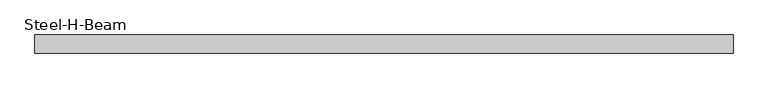
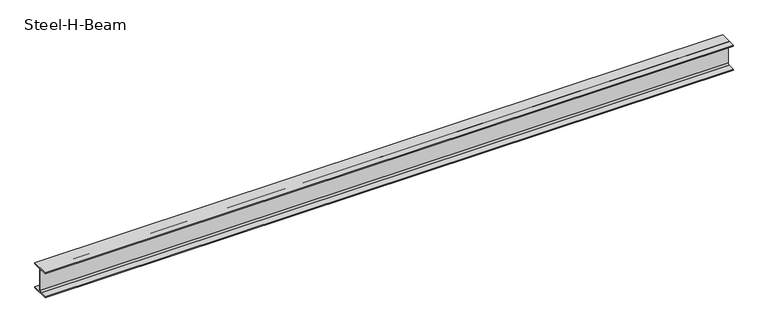
"""IFC4 building model written with IfcOpenShell, lengths in millimetres: beam geometry, Steel-H-Beam : BM121_H-294×200x8x12."""

from ifc_helpers import new_model, si_unit, point, frame, frame_2d, origin, place, context, project, spatial, polyline, circle_curve, trimmed, segment, composite_curve, outline, extrude, source, transform, mapped, element, save


def steel_h_beam_092dc31f(model_context):
    return source(origin(), model_context, "Body", "SweptSolid", [
        extrude(outline(composite_curve([segment(polyline([(100.0, -135.0), (100.0, -147.0), (-100.0, -147.0), (-100.0, -135.0), (-22.0, -135.0)]), True, "CONTINUOUS"), segment(trimmed(circle_curve(frame_2d((-22.0, -117.0)), 18.0), [point((-22.0, -135.0))], [point((-4.0, -117.0))], True, "CARTESIAN"), True, "CONTINUOUS"), segment(polyline([(-4.0, -117.0), (-4.0, 117.0)]), True, "CONTINUOUS"), segment(trimmed(circle_curve(frame_2d((-22.0, 117.0)), 18.0), [point((-4.0, 117.0))], [point((-22.0, 135.0))], True, "CARTESIAN"), True, "CONTINUOUS"), segment(polyline([(-22.0, 135.0), (-100.0, 135.0), (-100.0, 147.0), (100.0, 147.0), (100.0, 135.0), (22.0, 135.0)]), True, "CONTINUOUS"), segment(trimmed(circle_curve(frame_2d((22.0, 117.0)), 18.0), [point((22.0, 135.0))], [point((4.0, 117.0))], True, "CARTESIAN"), True, "CONTINUOUS"), segment(polyline([(4.0, 117.0), (4.0, -117.0)]), True, "CONTINUOUS"), segment(trimmed(circle_curve(frame_2d((22.0, -117.0)), 18.0), [point((4.0, -117.0))], [point((22.0, -135.0))], True, "CARTESIAN"), True, "CONTINUOUS"), segment(polyline([(22.0, -135.0), (100.0, -135.0)]), True, "CONTINUOUS")], self_intersect=False)), frame((-3684.2656766, 0.0, 0.0), z_axis=(1.0, 0.0, 0.0), x_axis=(0.0, 1.0, 0.0)), (0.0, 0.0, 1.0), 7684.2656766),
    ])


if __name__ == "__main__":
    model = new_model("IFC4")
    model_context = context("Model", 3, world=origin())
    ifc_project = project(units=[si_unit("LENGTHUNIT", "METRE", prefix="MILLI")], contexts=[model_context])
    site = spatial("IfcSite", under=ifc_project)
    building = spatial("IfcBuilding", under=site)
    placement = place(None, origin())
    steel_h_beam_shape = steel_h_beam_092dc31f(model_context)
    element("IfcBeam", 1, ObjectType="Steel-H-Beam : BM121_H-294×200x8x12", at=placement, inside=building, context=model_context, shape_type="MappedRepresentation", body=[
        mapped(steel_h_beam_shape, transform((0.0, 0.0, 0.0), x_axis=(1.0, 0.0, 0.0), y_axis=(0.0, 1.0, 0.0), z_axis=(0.0, 0.0, 1.0))),
    ])
    save(model, "model.ifc")

# Revit data of these elements
# Type "Steel-H-Beam : BM121_H-294×200x8x12"
#   Surface Area = 1.3411 m²/m
#   Section Area = 72.3812 cm²
#   Mass per Unit Length = 56.8193 kg/m
#   Length [instance default] = 3000 mm
#   B = 200 mm
#   H = 294 mm
#   r = 18 mm
#   tw = 8 mm
#   tf = 12 mm
#   hec_material4 [instance default] = none
#   hec_material3 [instance default] = none
#   hec_material2 [instance default] = none
#   hec_material1 [instance default] = none
#   Structural Material [instance default] = Steel, 45-345
#   Assembly Code = ""
# Element 1 (IfcBeam, "Steel-H-Beam : BM121_H-294×200x8x12")
#   hec_material3 = F01AC000-00002_Building/Shelter Fire Proofing Work_Intumescent Coating Type_1 hr. rating (UL 1709))
#   hec_material2 = S01AA010-00002_Main Steel Structure Fabrication Work_Shelter/Building_Steel Painting/Coating_for Fireproofed Steel Surface, Surface Preparation & Primer Coat
#   hec_material1 = S03AA028-00001_Main Steel Structure Erection Work_Shelter/Building_Medium Steel
#   Structural Material = S01AA002-00001_Main Steel Structure Fabrication Work_Shelter/Building_Medium Steel - Standard
#   Materials on its faces: "S01AA002-00001_Main Steel Structure Fabrication Work_Shelter/Building_Medium Steel - Standard"
# Materials
#   "Steel, 45-345": class "Metal", colour RGB 189 187 185, transparency 0, Description = "Steel 345 MPa", Cost = 0
#   "S01AA002-00001_Main Steel Structure Fabrication Work_Shelter/Building_Medium Steel - Standard": class "Metal", colour RGB 120 120 120, transparency 0, Comments = "(90KG/M>Weight≥30KG/M)", Description = "Structural steel 50ksi", W00) Work Master Code = "S01AA002-0001", W01) Work Master_Lv1 = "Main Steel Structure Fabrication Work", W02) Work Master_Lv2 = "Shelter/Building", W03) Work Master_Spec.1 = "Medium Steel - Standard (90KG/M>Weight≥30KG/M)", Cost = 0
#   "F01AC000-00002_Building/Shelter Fire Proofing Work_Intumescent Coating Type_1 hr. rating (UL 1709))": class "Metal", colour RGB 255 128 128, transparency 0, Description = "Paint finished steel", W00) Work Master Code = "F01AC000-00002", W01) Work Master_Lv1 = "Building/Shelter Fire Proofing Work", W02) Work Master_Lv2 = "Intumescent Coating Type", W03) Work Master_Spec.1 = "1 hr. rating (UL 1709)", Cost = 0
#   "S01AA010-00002_Main Steel Structure Fabrication Work_Shelter/Building_Steel Painting/Coating_for Fireproofed Steel Surface, Surface Preparation & Primer Coat": class "Metal", colour RGB 120 120 120, transparency 0, Description = "Paint finished steel", W00) Work Master Code = "SS01AA010-00002", W01) Work Master_Lv1 = "Main Steel Structure Fabrication Work", W02) Work Master_Lv2 = "Shelter/Building", W03) Work Master_Spec.1 = "Steel Painting/Coating", W04) Work Master_Spec.2 = "for Fireproofed Steel Surface, Surface Preparation & Primer Coat", Cost = 0
#   "S03AA028-00001_Main Steel Structure Erection Work_Shelter/Building_Medium Steel": class "Metal", colour RGB 120 120 120, transparency 0, Comments = "(90KG/M>Weight≥30KG/M)", Description = "Structural steel 50ksi", W00) Work Master Code = "S03AA028-0001", W01) Work Master_Lv1 = "Main Steel Structure Erection Work", W02) Work Master_Lv2 = "Shelter/Building", W03) Work Master_Spec.1 = "Medium Steel (90KG/M>Weight≥30KG/M)", Cost = 0
